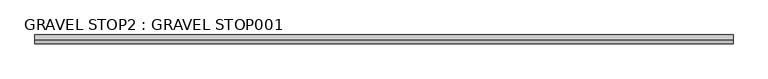
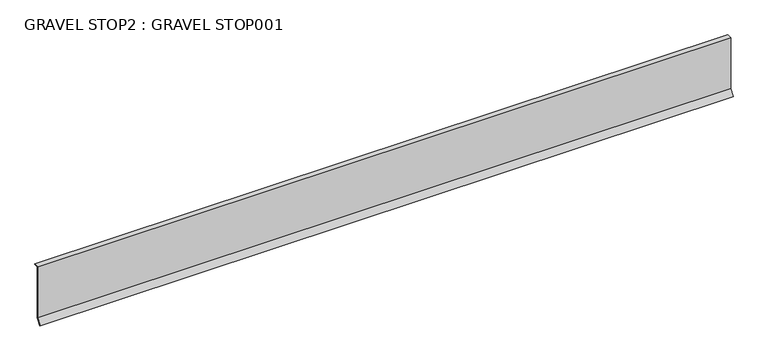
"""IFC4 building model written with IfcOpenShell, lengths in millimetres: proxy geometry, GRAVEL STOP2 : GRAVEL STOP001."""

from ifc_helpers import new_model, si_unit, frame, origin, place, context, project, spatial, polyline, outline, extrude, source, transform, mapped, element, save


def gravel_stop2_gravel_stop001_6aa894b6(model_context):
    return source(origin(), model_context, "Body", "SweptSolid", [
        extrude(outline(polyline([(-5588.2594715, 40065.903984), (-5575.6959005, 40081.6491197), (-5575.6959005, 40238.3989826), (-5562.5168708, 40238.3989826), (-5562.5168708, 40236.9878716), (-5574.2847895, 40236.9878716), (-5574.2847895, 40081.1551279), (-5587.1564679, 40065.0238605), (-5588.2594715, 40065.903984)])), frame((12382.7678845, 0.0, 0.0), z_axis=(1.0, 0.0, 0.0), x_axis=(0.0, 1.0, 0.0)), (0.0, 0.0, 1.0), 2000.25),
    ])


if __name__ == "__main__":
    model = new_model("IFC4")
    model_context = context("Model", 3, world=origin())
    ifc_project = project(units=[si_unit("LENGTHUNIT", "METRE", prefix="MILLI")], contexts=[model_context])
    site = spatial("IfcSite", under=ifc_project)
    building = spatial("IfcBuilding", under=site)
    placement = place(None, origin())
    gravel_stop2_gravel_stop001_shape = gravel_stop2_gravel_stop001_6aa894b6(model_context)
    element("IfcBuildingElementProxy", 1, Name="GRAVEL STOP2 : GRAVEL STOP001", ObjectType="GRAVEL STOP2 : GRAVEL STOP001", at=placement, inside=building, context=model_context, shape_type="MappedRepresentation", body=[
        mapped(gravel_stop2_gravel_stop001_shape, transform((0.0, 0.0, 0.0), x_axis=(1.0, 0.0, 0.0), y_axis=(0.0, 1.0, 0.0), z_axis=(0.0, 0.0, 1.0))),
    ])
    save(model, "model.ifc")

# Revit data of these elements
# Type "GRAVEL STOP2 : GRAVEL STOP001"
#   NameOverride = "GRAVEL STOP001"
# Element 1 (IfcBuildingElementProxy, "GRAVEL STOP2 : GRAVEL STOP001")
#   Materials on its faces: "GRAVEL STOP REQUIRED WITH GRAVEL SURFACE SYSTEMS"
# Materials
#   "GRAVEL STOP REQUIRED WITH GRAVEL SURFACE SYSTEMS": class "Unassigned", colour RGB 170 170 127, transparency 0, Cost = 0
